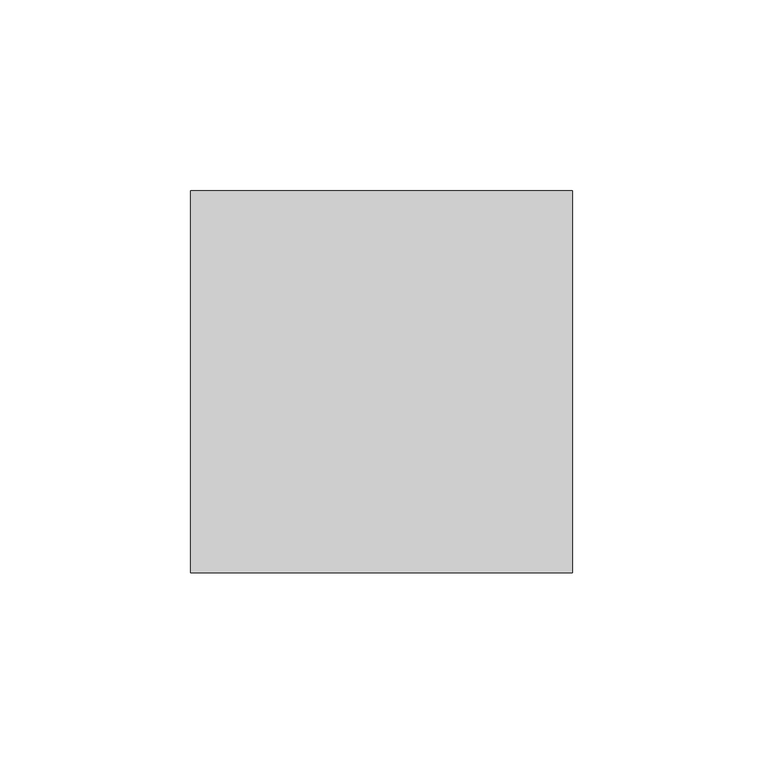
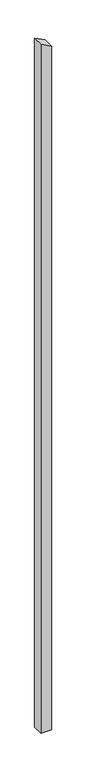
"""IFC4 building model written with IfcOpenShell, lengths in millimetres: column geometry, Holzstütze 159256 : Holzstütze 159256."""

import ifcopenshell
import ifcopenshell.guid

model = None  # the IFC model being written
_history = None  # IfcOwnerHistory: only IFC2X3 demands one
_inside = {}  # id of a spatial element -> (the spatial element, [elements in it])
_under = {}  # id of a project, library or spatial element -> (it, [spatial elements below it])
_declared = {}  # id of a project -> (the project, [libraries it declares])
_typed = {}  # id of a type object -> (the type object, [elements of that type])
_made_of = {}  # id of a material, layer set ... -> (it, [elements and type objects made of it])


def new_model(schema):
    """Start an empty IFC model of exactly this schema.

    Asked for "IFC4X3", IfcOpenShell would pick the latest addendum, in which some entities
    have other attributes; the version numbers below select the first issue.
    IFC2X3 requires an IfcOwnerHistory on every rooted entity: one is made here for all.
    """
    global model, _history
    if schema == "IFC4X3":
        model = ifcopenshell.file(schema_version=(4, 3, 0, 0))
    else:
        model = ifcopenshell.file(schema=schema)
    _inside.clear()
    _under.clear()
    _declared.clear()
    _typed.clear()
    _made_of.clear()
    _history = None
    if model.schema == "IFC2X3":
        org = make("IfcOrganization", Name="unknown")
        user = make(
            "IfcPersonAndOrganization",
            ThePerson=make("IfcPerson", FamilyName="unknown"),
            TheOrganization=org,
        )
        app = make(
            "IfcApplication",
            ApplicationDeveloper=org,
            Version="unknown",
            ApplicationFullName="unknown",
            ApplicationIdentifier="unknown",
        )
        _history = make(
            "IfcOwnerHistory",
            OwningUser=user,
            OwningApplication=app,
            ChangeAction="ADDED",
            CreationDate=0,
        )
    return model


def make(cls, **values):
    """One entity of the class cls with the attributes given. An attribute that is None is left unset."""
    return model.create_entity(
        cls, **{name: value for name, value in values.items() if value is not None}
    )


def rooted(cls, **values):
    """An entity with a GlobalId (a new one), such as an element, a storey or a relation."""
    return make(cls, GlobalId=ifcopenshell.guid.new(), OwnerHistory=_history, **values)


def si_unit(unit_type, name, prefix=None):
    """IfcSIUnit, for example si_unit("LENGTHUNIT", "METRE", prefix="MILLI")."""
    return make("IfcSIUnit", UnitType=unit_type, Prefix=prefix, Name=name)


def assignment(units):
    """IfcUnitAssignment: the units of a project."""
    return None if units is None else make("IfcUnitAssignment", Units=units)


def point(xyz):
    """IfcCartesianPoint."""
    return None if xyz is None else make("IfcCartesianPoint", Coordinates=xyz)


def direction(xyz):
    """IfcDirection."""
    return None if xyz is None else make("IfcDirection", DirectionRatios=xyz)


def frame(location, z_axis=None, x_axis=None):
    """IfcAxis2Placement3D, a coordinate frame: its origin and axes. An axis left out is left unset."""
    return make(
        "IfcAxis2Placement3D",
        Location=point(location),
        Axis=direction(z_axis),
        RefDirection=direction(x_axis),
    )


def origin():
    """The frame at (0, 0, 0) with its axes left unset."""
    return frame((0.0, 0.0, 0.0))


def place(relative_to, where):
    """IfcLocalPlacement: puts the frame where relative to a parent placement (None: the world)."""
    return make(
        "IfcLocalPlacement", PlacementRelTo=relative_to, RelativePlacement=where
    )


def context(
    kind, dimensions, precision=None, world=None, true_north=None, identifier=None
):
    """IfcGeometricRepresentationContext, for example the 3D "Model" context."""
    return make(
        "IfcGeometricRepresentationContext",
        ContextIdentifier=identifier,
        ContextType=kind,
        CoordinateSpaceDimension=dimensions,
        Precision=precision,
        WorldCoordinateSystem=world,
        TrueNorth=true_north,
    )


def project(units=None, contexts=None):
    """IfcProject with its units and contexts."""
    return rooted(
        "IfcProject",
        Name="project",
        RepresentationContexts=contexts,
        UnitsInContext=assignment(units),
    )


def spatial(cls, under=None, at=None, **own):
    """A site, building, storey or space (cls), placed at a placement, below another one or the project."""
    s = rooted(cls, ObjectPlacement=at, **own)
    if under is not None:
        _under.setdefault(under.id(), (under, []))[1].append(s)
    return s


def polyline(points):
    """IfcPolyline through the points."""
    return make("IfcPolyline", Points=[point(p) for p in points])


def outline(outer, holes=None, kind="AREA"):
    """IfcArbitraryClosedProfileDef: a profile drawn as a closed curve; with holes, ...WithVoids."""
    if holes is None:
        return make("IfcArbitraryClosedProfileDef", ProfileType=kind, OuterCurve=outer)
    return make(
        "IfcArbitraryProfileDefWithVoids",
        ProfileType=kind,
        OuterCurve=outer,
        InnerCurves=holes,
    )


def extrude(swept, where, along, depth):
    """IfcExtrudedAreaSolid: the profile swept, set in the frame where, extruded along a direction by depth."""
    return make(
        "IfcExtrudedAreaSolid",
        SweptArea=swept,
        Position=where,
        ExtrudedDirection=direction(along),
        Depth=depth,
    )


def shape(context_of_items, identifier, shape_type, items):
    """IfcShapeRepresentation: the items that make up one representation, for example the "Body"."""
    return make(
        "IfcShapeRepresentation",
        ContextOfItems=context_of_items,
        RepresentationIdentifier=identifier,
        RepresentationType=shape_type,
        Items=items,
    )


def source(mapping_origin, context_of_items, identifier, shape_type, items):
    """IfcRepresentationMap: a shape defined once, which mapped items show again and again."""
    return make(
        "IfcRepresentationMap",
        MappingOrigin=mapping_origin,
        MappedRepresentation=shape(context_of_items, identifier, shape_type, items),
    )


def transform(
    local_origin,
    x_axis=None,
    y_axis=None,
    z_axis=None,
    scale=None,
    scale2=None,
    scale3=None,
    uniform=True,
):
    """IfcCartesianTransformationOperator3D, or its non-uniform kind. x_axis, y_axis, z_axis: its Axis1, 2, 3."""
    if uniform:
        return make(
            "IfcCartesianTransformationOperator3D",
            Axis1=direction(x_axis),
            Axis2=direction(y_axis),
            LocalOrigin=point(local_origin),
            Scale=scale,
            Axis3=direction(z_axis),
        )
    return make(
        "IfcCartesianTransformationOperator3DnonUniform",
        Axis1=direction(x_axis),
        Axis2=direction(y_axis),
        LocalOrigin=point(local_origin),
        Scale=scale,
        Axis3=direction(z_axis),
        Scale2=scale2,
        Scale3=scale3,
    )


def mapped(mapping_source, mapping_target):
    """IfcMappedItem: shows the shape of a source again, moved by a transform."""
    return make(
        "IfcMappedItem", MappingSource=mapping_source, MappingTarget=mapping_target
    )


def made_of(thing, what):
    """Note that an element or type object is made of a material, layer set ...; save() writes the relation."""
    if what is not None:
        _made_of.setdefault(what.id(), (what, []))[1].append(thing)
    return thing


def element(
    cls,
    number,
    at=None,
    inside=None,
    cuts=None,
    type_object=None,
    material=None,
    context=None,
    identifier="Body",
    shape_type=None,
    held_by="IfcProductDefinitionShape",
    body=None,
    shapes=None,
    **own,
):
    """One element of the class cls, such as IfcWall. Its Tag is "e" and its number.

    at: its placement. inside: the storey or other place that contains it. cuts: it is an
    opening in that element (IfcRelVoidsElement). A single representation is given by context,
    identifier, shape_type and body (its items); several are given by shapes. held_by: the class
    of the entity that holds the representations. save() writes the other relations.
    """
    e = rooted(cls, Tag="e%d" % number, ObjectPlacement=at, **own)
    if body is not None:
        shapes = [shape(context, identifier, shape_type, body)]
    if shapes is not None:
        e.Representation = make(held_by, Representations=shapes)
    if inside is not None:
        _inside.setdefault(inside.id(), (inside, []))[1].append(e)
    if cuts is not None:
        rooted(
            "IfcRelVoidsElement", RelatingBuildingElement=cuts, RelatedOpeningElement=e
        )
    if type_object is not None:
        _typed.setdefault(type_object.id(), (type_object, []))[1].append(e)
    return made_of(e, material)


def aggregate(whole, parts):
    """IfcRelAggregates: a whole, such as a stair, and the parts it consists of."""
    return rooted("IfcRelAggregates", RelatingObject=whole, RelatedObjects=parts)


def save(model, path):
    """Write the relations noted so far, then the file.

    IfcRelAggregates (storeys below a building ...), IfcRelContainedInSpatialStructure (elements
    in a storey), IfcRelDefinesByType, IfcRelAssociatesMaterial and IfcRelDeclares: one each for
    every whole, place, type object, material and project.
    """
    for whole, parts in _under.values():
        aggregate(whole, parts)
    for where, things in _inside.values():
        rooted(
            "IfcRelContainedInSpatialStructure",
            RelatedElements=things,
            RelatingStructure=where,
        )
    for kind, things in _typed.values():
        rooted("IfcRelDefinesByType", RelatedObjects=things, RelatingType=kind)
    for what, things in _made_of.values():
        rooted("IfcRelAssociatesMaterial", RelatedObjects=things, RelatingMaterial=what)
    for by, libraries in _declared.values():
        rooted("IfcRelDeclares", RelatingContext=by, RelatedDefinitions=libraries)
    model.write(path)


def column_b6b0c2fc(model_context):
    return source(origin(), model_context, "Body", "SweptSolid", [
        extrude(outline(polyline([(-500.0, 174197.7593015), (-500.0, 174297.7593015), (6345.7118258, 174297.7593015), (6396.6643707, 174197.7593015), (-500.0, 174197.7593015)])), frame((0.0, 36959.3988814, 0.0), z_axis=(0.0, 1.0, 0.0), x_axis=(0.0, 0.0, 1.0)), (0.0, 0.0, 1.0), 100.0),
    ])


if __name__ == "__main__":
    model = new_model("IFC4")
    model_context = context("Model", 3, world=origin())
    ifc_project = project(units=[si_unit("LENGTHUNIT", "METRE", prefix="MILLI")], contexts=[model_context])
    site = spatial("IfcSite", under=ifc_project)
    building = spatial("IfcBuilding", under=site)
    placement = place(None, origin())
    column_shape = column_b6b0c2fc(model_context)
    element("IfcColumn", 1, ObjectType="Holzstütze 159256 : Holzstütze 159256", at=placement, inside=building, context=model_context, shape_type="MappedRepresentation", body=[
        mapped(column_shape, transform((0.0, 0.0, 0.0), x_axis=(1.0, 0.0, 0.0), y_axis=(0.0, 1.0, 0.0), z_axis=(0.0, 0.0, 1.0))),
    ])
    save(model, "model.ifc")

# Revit data of these elements
# Type "Holzstütze 159256 : Holzstütze 159256"
#   Abrechnungsart = "m"
#   Allright_Bauteil_ID = "0152St 0000143356"
#   Bezeichnung = "Holzstütze"
#   Codetext = "ST-HOLZ\\"
#   Gewerk = "Zimmer- und Holzbauarbeiten"
#   Material = "Holz"
#   Objektname = "Stütze"
#   NameOverride = "Holzstütze"
#   Reference = "Holzstütze"
#   Status = "NEW"
#   ThermalTransmittance = 0.0000 BTU/(h·ft²·°F)
#   Roll = 0.00°
#   Slope = 0.00°
#   2D Interaktion = yes
#   IsExternal = yes
#   LoadBearing = yes
# Element 1 (IfcColumn, "Holzstütze 159256 : Holzstütze 159256")
#   Materials on its faces: "holzschalung"
# Materials
#   "holzschalung": class "Unassigned", colour RGB 128 128 128, transparency 0
